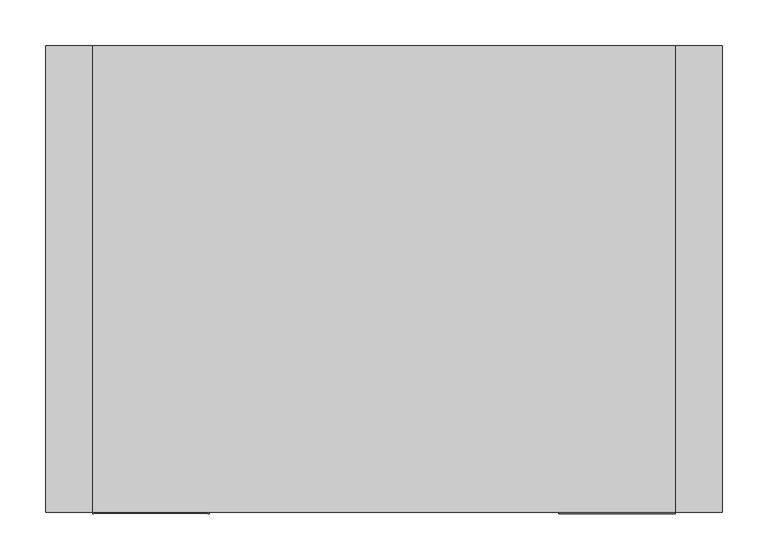
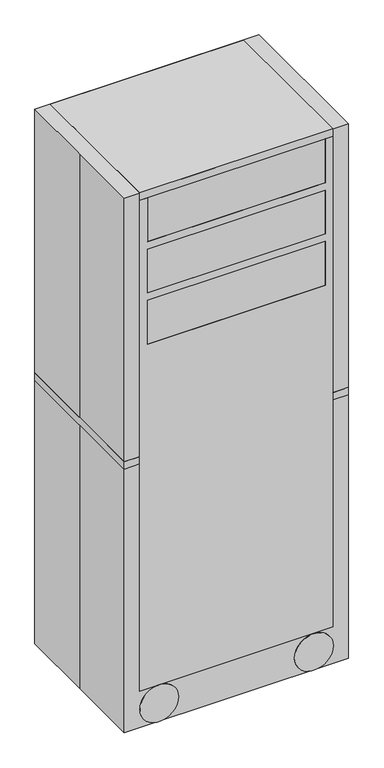
"""IFC4 building model written with IfcOpenShell, lengths in millimetres: proxy geometry, E0930 - Locker, Supply, 6 Drawers, Mobile, 29W x 20D : E0930 - Locker, Supply, 6 Drawers, Mobile, 29W x 20D."""

from ifc_helpers import new_model, si_unit, point, frame, frame_2d, origin, origin_with_axes, place, context, project, spatial, polyline, circle_curve, trimmed, segment, composite_curve, outline, extrude, source, transform, mapped, element, save
from ifc_brep_helpers import plane_surface, cylinder_surface, advanced_brep


def specialty_equipment_c401bbb8(model_context):
    return source(origin(), model_context, "Body", "SolidModel", [
        extrude(outline(polyline([(317.5, -254.0), (-317.5, -254.0), (-317.5, 254.0), (317.5, 254.0), (317.5, -254.0)])), frame((0.0, 0.0, 1828.8), z_axis=(0.0, 0.0, 1.0), x_axis=(1.0, 0.0, 0.0)), (0.0, 0.0, 1.0), 25.4),
        extrude(outline(composite_curve([segment(trimmed(circle_curve(frame_2d((-275.1666667, -206.375)), 21.1666667), [point((-275.1666667, -227.5416667))], [point((-275.1666667, -185.2083333))], False, "CARTESIAN"), True, "CONTINUOUS"), segment(trimmed(circle_curve(frame_2d((-275.1666667, -206.375)), 21.1666667), [point((-275.1666667, -185.2083333))], [point((-275.1666667, -227.5416667))], False, "CARTESIAN"), True, "CONTINUOUS")], self_intersect=False)), frame((0.0, 0.0, 53.8442082), z_axis=(0.0, 0.0, 1.0), x_axis=(1.0, 0.0, 0.0)), (0.0, 0.0, 1.0), 73.1557918),
        extrude(outline(composite_curve([segment(trimmed(circle_curve(frame_2d((63.5, -254.0)), 42.3333333), [point((63.5, -211.6666667))], [point((63.5, -296.3333333))], False, "CARTESIAN"), True, "CONTINUOUS"), segment(trimmed(circle_curve(frame_2d((63.5, -254.0)), 42.3333333), [point((63.5, -296.3333333))], [point((63.5, -211.6666667))], False, "CARTESIAN"), True, "CONTINUOUS")], self_intersect=False)), frame((0.0, -231.2458333, 0.0), z_axis=(0.0, 1.0, 0.0), x_axis=(0.0, 0.0, 1.0)), (0.0, 0.0, 1.0), 47.625),
        extrude(outline(composite_curve([segment(trimmed(circle_curve(frame_2d((63.5, -254.0)), 63.5), [point((63.5, -190.5))], [point((63.5, -317.5))], False, "CARTESIAN"), True, "CONTINUOUS"), segment(trimmed(circle_curve(frame_2d((63.5, -254.0)), 63.5), [point((63.5, -317.5))], [point((63.5, -190.5))], False, "CARTESIAN"), True, "CONTINUOUS")], self_intersect=False)), frame((0.0, -255.0583333, 0.0), z_axis=(0.0, 1.0, 0.0), x_axis=(0.0, 0.0, 1.0)), (0.0, 0.0, 1.0), 23.8125),
        extrude(outline(composite_curve([segment(trimmed(circle_curve(frame_2d((63.5, -254.0)), 63.5), [point((63.5, -190.5))], [point((63.5, -317.5))], False, "CARTESIAN"), True, "CONTINUOUS"), segment(trimmed(circle_curve(frame_2d((63.5, -254.0)), 63.5), [point((63.5, -317.5))], [point((63.5, -190.5))], False, "CARTESIAN"), True, "CONTINUOUS")], self_intersect=False)), frame((0.0, -183.6208333, 0.0), z_axis=(0.0, 1.0, 0.0), x_axis=(0.0, 0.0, 1.0)), (0.0, 0.0, 1.0), 23.8125),
        extrude(outline(composite_curve([segment(trimmed(circle_curve(frame_2d((275.1666667, -206.375)), 21.1666667), [point((275.1666667, -227.5416667))], [point((275.1666667, -185.2083333))], False, "CARTESIAN"), True, "CONTINUOUS"), segment(trimmed(circle_curve(frame_2d((275.1666667, -206.375)), 21.1666667), [point((275.1666667, -185.2083333))], [point((275.1666667, -227.5416667))], False, "CARTESIAN"), True, "CONTINUOUS")], self_intersect=False)), frame((0.0, 0.0, 53.8442082), z_axis=(0.0, 0.0, 1.0), x_axis=(1.0, 0.0, 0.0)), (0.0, 0.0, 1.0), 73.1557918),
        extrude(outline(composite_curve([segment(trimmed(circle_curve(frame_2d((63.5, 254.0)), 42.3333333), [point((63.5, 211.6666667))], [point((63.5, 296.3333333))], False, "CARTESIAN"), True, "CONTINUOUS"), segment(trimmed(circle_curve(frame_2d((63.5, 254.0)), 42.3333333), [point((63.5, 296.3333333))], [point((63.5, 211.6666667))], False, "CARTESIAN"), True, "CONTINUOUS")], self_intersect=False)), frame((0.0, -231.775, 0.0), z_axis=(0.0, 1.0, 0.0), x_axis=(0.0, 0.0, 1.0)), (0.0, 0.0, 1.0), 47.625),
        extrude(outline(composite_curve([segment(trimmed(circle_curve(frame_2d((63.5, 254.0)), 63.5), [point((63.5, 190.5))], [point((63.5, 317.5))], False, "CARTESIAN"), True, "CONTINUOUS"), segment(trimmed(circle_curve(frame_2d((63.5, 254.0)), 63.5), [point((63.5, 317.5))], [point((63.5, 190.5))], False, "CARTESIAN"), True, "CONTINUOUS")], self_intersect=False)), frame((0.0, -255.5875, 0.0), z_axis=(0.0, 1.0, 0.0), x_axis=(0.0, 0.0, 1.0)), (0.0, 0.0, 1.0), 23.8125),
        extrude(outline(composite_curve([segment(trimmed(circle_curve(frame_2d((63.5, 254.0)), 63.5), [point((63.5, 190.5))], [point((63.5, 317.5))], False, "CARTESIAN"), True, "CONTINUOUS"), segment(trimmed(circle_curve(frame_2d((63.5, 254.0)), 63.5), [point((63.5, 317.5))], [point((63.5, 190.5))], False, "CARTESIAN"), True, "CONTINUOUS")], self_intersect=False)), frame((0.0, -184.15, 0.0), z_axis=(0.0, 1.0, 0.0), x_axis=(0.0, 0.0, 1.0)), (0.0, 0.0, 1.0), 23.8125),
        extrude(outline(composite_curve([segment(trimmed(circle_curve(frame_2d((-275.1666667, 206.375)), 21.1666667), [point((-275.1666667, 227.5416667))], [point((-275.1666667, 185.2083333))], False, "CARTESIAN"), True, "CONTINUOUS"), segment(trimmed(circle_curve(frame_2d((-275.1666667, 206.375)), 21.1666667), [point((-275.1666667, 185.2083333))], [point((-275.1666667, 227.5416667))], False, "CARTESIAN"), True, "CONTINUOUS")], self_intersect=False)), frame((0.0, 0.0, 53.8442082), z_axis=(0.0, 0.0, 1.0), x_axis=(1.0, 0.0, 0.0)), (0.0, 0.0, 1.0), 73.1557918),
        extrude(outline(composite_curve([segment(trimmed(circle_curve(frame_2d((63.5, -254.0)), 42.3333333), [point((63.5, -211.6666667))], [point((63.5, -296.3333333))], False, "CARTESIAN"), True, "CONTINUOUS"), segment(trimmed(circle_curve(frame_2d((63.5, -254.0)), 42.3333333), [point((63.5, -296.3333333))], [point((63.5, -211.6666667))], False, "CARTESIAN"), True, "CONTINUOUS")], self_intersect=False)), frame((0.0, 182.5625, 0.0), z_axis=(0.0, 1.0, 0.0), x_axis=(0.0, 0.0, 1.0)), (0.0, 0.0, 1.0), 47.625),
        extrude(outline(composite_curve([segment(trimmed(circle_curve(frame_2d((63.5, -254.0)), 63.5), [point((63.5, -190.5))], [point((63.5, -317.5))], False, "CARTESIAN"), True, "CONTINUOUS"), segment(trimmed(circle_curve(frame_2d((63.5, -254.0)), 63.5), [point((63.5, -317.5))], [point((63.5, -190.5))], False, "CARTESIAN"), True, "CONTINUOUS")], self_intersect=False)), frame((0.0, 230.1875, 0.0), z_axis=(0.0, 1.0, 0.0), x_axis=(0.0, 0.0, 1.0)), (0.0, 0.0, 1.0), 23.8125),
        extrude(outline(composite_curve([segment(trimmed(circle_curve(frame_2d((63.5, -254.0)), 63.5), [point((63.5, -190.5))], [point((63.5, -317.5))], False, "CARTESIAN"), True, "CONTINUOUS"), segment(trimmed(circle_curve(frame_2d((63.5, -254.0)), 63.5), [point((63.5, -317.5))], [point((63.5, -190.5))], False, "CARTESIAN"), True, "CONTINUOUS")], self_intersect=False)), frame((0.0, 158.75, 0.0), z_axis=(0.0, 1.0, 0.0), x_axis=(0.0, 0.0, 1.0)), (0.0, 0.0, 1.0), 23.8125),
        advanced_brep(
        [(275.1666667, 227.5416667, 127.0), (275.1666667, 185.2083333, 127.0), (275.1666667, 227.5416667, 53.8442082), (295.2174332, 213.1569275, 53.8442082), (275.1666667, 185.2083333, 53.8442082), (254.0596152, 207.9625, 53.8442082), (275.1666667, 227.5416667, 100.1617421)],
        [
            (0, 1, circle_curve(frame((275.1666667, 206.375, 127.0), z_axis=(0.0, 0.0, 1.0), x_axis=(0.0, -1.0, 0.0)), 21.1666667)),
            (1, 0, circle_curve(frame((275.1666667, 206.375, 127.0), z_axis=(0.0, 0.0, 1.0), x_axis=(0.0, -1.0, 0.0)), 21.1666667)),
            (2, 3, circle_curve(frame((275.1666667, 206.375, 53.8442082), z_axis=(0.0, 0.0, -1.0), x_axis=(0.0, -1.0, 0.0)), 21.1666667)),
            (3, 4, circle_curve(frame((275.1666667, 206.375, 53.8442082), z_axis=(0.0, 0.0, -1.0), x_axis=(0.0, -1.0, 0.0)), 21.1666667)),
            (4, 5, circle_curve(frame((275.1666667, 206.375, 53.8442082), z_axis=(0.0, 0.0, -1.0), x_axis=(0.0, -1.0, 0.0)), 21.1666667)),
            (5, 2, circle_curve(frame((275.1666667, 206.375, 53.8442082), z_axis=(0.0, 0.0, -1.0), x_axis=(0.0, -1.0, 0.0)), 21.1666667)),
            (0, 6),
            (6, 2),
            (4, 1),
        ],
        [
            plane_surface(frame((275.1666667, 185.2083333, 127.0), z_axis=(0.0, 0.0, 1.0), x_axis=(1.0, 0.0, 0.0))),
            plane_surface(frame((275.1666667, 185.2083333, 53.8442082), z_axis=(0.0, 0.0, -1.0), x_axis=(-1.0, 0.0, 0.0))),
            cylinder_surface(frame((275.1666667, 206.375, 53.8442082), z_axis=(0.0, 0.0, 1.0), x_axis=(0.0, -1.0, 0.0)), 21.1666667),
        ],
        [
            (0, [[1, 2]]),
            (1, [[3, 4, 5, 6]]),
            (2, [[-1, 7, 8, -6, -5, 9]]),
            (2, [[-2, -9, -4, -3, -8, -7]]),
        ],
    ),
        extrude(outline(composite_curve([segment(trimmed(circle_curve(frame_2d((63.5, 254.0)), 63.5), [point((63.5, 190.5))], [point((63.5, 317.5))], False, "CARTESIAN"), True, "CONTINUOUS"), segment(trimmed(circle_curve(frame_2d((63.5, 254.0)), 63.5), [point((63.5, 317.5))], [point((63.5, 190.5))], False, "CARTESIAN"), True, "CONTINUOUS")], self_intersect=False)), frame((0.0, 230.1875, 0.0), z_axis=(0.0, 1.0, 0.0), x_axis=(0.0, 0.0, 1.0)), (0.0, 0.0, 1.0), 23.8125),
        extrude(outline(composite_curve([segment(trimmed(circle_curve(frame_2d((63.5, 254.0)), 63.5), [point((63.5, 190.5))], [point((63.5, 317.5))], False, "CARTESIAN"), True, "CONTINUOUS"), segment(trimmed(circle_curve(frame_2d((63.5, 254.0)), 63.5), [point((63.5, 317.5))], [point((63.5, 190.5))], False, "CARTESIAN"), True, "CONTINUOUS")], self_intersect=False)), frame((0.0, 158.75, 0.0), z_axis=(0.0, 1.0, 0.0), x_axis=(0.0, 0.0, 1.0)), (0.0, 0.0, 1.0), 23.8125),
        extrude(outline(polyline([(127.0, -317.5), (127.0, 317.5), (1828.8, 317.5), (1828.8, 292.1), (1676.4, 292.1), (1676.4, -292.1), (1828.8, -292.1), (1828.8, -317.5), (127.0, -317.5)]), holes=[polyline([(1651.0, -292.1), (1651.0, 292.1), (1498.6, 292.1), (1498.6, -292.1), (1651.0, -292.1)]), polyline([(1473.2, -292.1), (1473.2, 292.1), (1320.8, 292.1), (1320.8, -292.1), (1473.2, -292.1)])]), frame((0.0, -254.0, 0.0), z_axis=(0.0, 1.0, 0.0), x_axis=(0.0, 0.0, 1.0)), (0.0, 0.0, 1.0), 508.0),
        extrude(outline(polyline([(368.3, 254.0), (368.3, -254.0), (317.5, -254.0), (317.5, -228.6), (342.9, -228.6), (342.9, 228.6), (317.5, 228.6), (317.5, 254.0), (368.3, 254.0)])), frame((0.0, 0.0, 914.4), z_axis=(0.0, 0.0, 1.0), x_axis=(1.0, 0.0, 0.0)), (0.0, 0.0, 1.0), 25.4),
        extrude(outline(polyline([(-368.3, 254.0), (-317.5, 254.0), (-317.5, 228.6), (-342.9, 228.6), (-342.9, -228.6), (-317.5, -228.6), (-317.5, -254.0), (-368.3, -254.0), (-368.3, 254.0)])), frame((0.0, 0.0, 914.4), z_axis=(0.0, 0.0, 1.0), x_axis=(1.0, 0.0, 0.0)), (0.0, 0.0, 1.0), 25.4),
        extrude(outline(polyline([(-368.3, 254.0), (368.3, 254.0), (368.3, -254.0), (-368.3, -254.0), (-368.3, 0.0), (-368.3, 254.0)])), origin_with_axes(), (0.0, 0.0, 1.0), 1854.2),
    ])


if __name__ == "__main__":
    model = new_model("IFC4")
    model_context = context("Model", 3, world=origin())
    ifc_project = project(units=[si_unit("LENGTHUNIT", "METRE", prefix="MILLI")], contexts=[model_context])
    site = spatial("IfcSite", under=ifc_project)
    building = spatial("IfcBuilding", under=site)
    placement = place(None, origin())
    specialty_equipment_shape = specialty_equipment_c401bbb8(model_context)
    element("IfcBuildingElementProxy", 1, Name="E0930 - Locker, Supply, 6 Drawers, Mobile, 29W x 20D : E0930 - Locker, Supply, 6 Drawers, Mobile, 29W x 20D", ObjectType="E0930 - Locker, Supply, 6 Drawers, Mobile, 29W x 20D : E0930 - Locker, Supply, 6 Drawers, Mobile, 29W x 20D", at=placement, inside=building, context=model_context, shape_type="MappedRepresentation", body=[
        mapped(specialty_equipment_shape, transform((0.0, 0.0, 0.0), x_axis=(1.0, 0.0, 0.0), y_axis=(0.0, 1.0, 0.0), z_axis=(0.0, 0.0, 1.0))),
    ])
    save(model, "model.ifc")

# Revit data of these elements
# Type "E0930 - Locker, Supply, 6 Drawers, Mobile, 29W x 20D : E0930 - Locker, Supply, 6 Drawers, Mobile, 29W x 20D"
#   Watts2 = "0"
#   Watts1 = "0"
#   Unit_Issue = "EA"
#   UTIL_6_Misc = "-"
#   UTIL_5_NonMedGas = "-"
#   UTIL_4_MiscGas = "-"
#   UTIL_3_MedGas = "-"
#   UTIL_2_Elec = "-"
#   UTIL_1_WaterDrain = "-"
#   Nomenclature = "Locker, Supply, 6 Drawers, Mobile, 29\"W x 20\"D"
#   NSN = "6530"
#   Location [instance default] = ""
#   JSN = "E0930"
#   Fund_Source_VA = "V"
#   Fund_Source_Navy = "C"
#   Fund_Source_Army = "C"
#   Fund_Source_AF = "C"
#   ELEC_Volts2 = "0"
#   ELEC_Volts1 = "0"
#   ELEC_Phase2 = "0"
#   ELEC_Phase1 = "0"
#   ELEC_HertzSwitch = "0"
#   ELEC_HertzDependent = "0"
#   ELEC_Hertz = "0"
#   ELEC_Amps2 = "0"
#   ELEC_Amps1 = "0"
#   DetailDescription = "THIS TYPICAL INCLUDES:1 Mobile Supply Locker; 2 Tray/Shelf; 4 Drawers, 3\"H (76mm); 2 Drawers, 6\"H (152mm); Drawer Organizer Bins"
#   CAT_VA = "C"
#   CAT_Navy = "C"
#   CAT_IHS = "-"
#   CAT_Army = "C"
#   CAT_AF = "C"
#   BTUperhour = "0"
#   Weight_IP = 101
#   DIM_Width_IP = 2' - 5"
#   DIM_Height_IP = 6' - 1"
#   DIM_Depth_IP = 1' - 8"
#   finish [instance default] = none
# Element 1 (IfcBuildingElementProxy, "E0930 - Locker, Supply, 6 Drawers, Mobile, 29W x 20D : E0930 - Locker, Supply, 6 Drawers, Mobile, 29W x 20D")
#   Location = "TRPE1"
#   Materials on its faces: "EquipSpace"
# Materials
#   "EquipSpace": class "Unassigned", colour RGB 221 217 195, transparency 0.5
